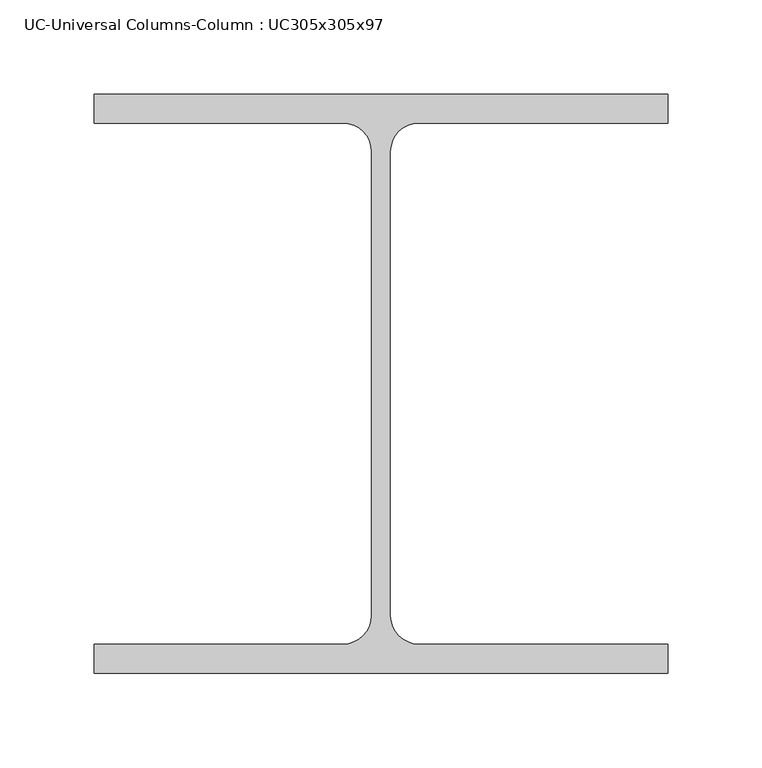
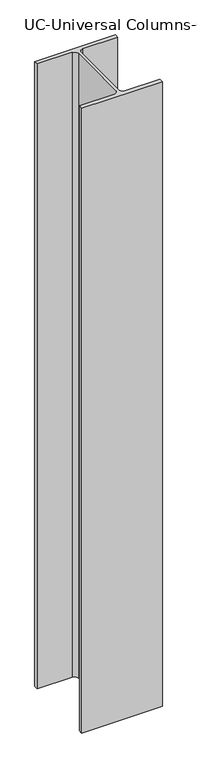
"""IFC4 building model written with IfcOpenShell, lengths in millimetres: column geometry, UC-Universal Columns-Column : UC305x305x97."""

from ifc_helpers import new_model, si_unit, point, frame_2d, origin, origin_with_axes, place, context, project, spatial, polyline, circle_curve, trimmed, segment, composite_curve, outline, extrude, source, transform, mapped, element, save


def uc_universal_columns_column_uc305x305x97_3ae92ab7(model_context):
    return source(origin(), model_context, "Body", "SweptSolid", [
        extrude(outline(composite_curve([segment(polyline([(152.65, 153.95), (152.65, 138.55), (20.15, 138.55)]), True, "CONTINUOUS"), segment(trimmed(circle_curve(frame_2d((20.15, 123.35)), 15.2), [point((20.15, 138.55))], [point((4.95, 123.35))], True, "CARTESIAN"), True, "CONTINUOUS"), segment(polyline([(4.95, 123.35), (4.95, -123.35)]), True, "CONTINUOUS"), segment(trimmed(circle_curve(frame_2d((20.15, -123.35)), 15.2), [point((4.95, -123.35))], [point((20.15, -138.55))], True, "CARTESIAN"), True, "CONTINUOUS"), segment(polyline([(20.15, -138.55), (152.65, -138.55), (152.65, -153.95), (-152.65, -153.95), (-152.65, -138.55), (-20.15, -138.55)]), True, "CONTINUOUS"), segment(trimmed(circle_curve(frame_2d((-20.15, -123.35)), 15.2), [point((-20.15, -138.55))], [point((-4.95, -123.35))], True, "CARTESIAN"), True, "CONTINUOUS"), segment(polyline([(-4.95, -123.35), (-4.95, 123.35)]), True, "CONTINUOUS"), segment(trimmed(circle_curve(frame_2d((-20.15, 123.35)), 15.2), [point((-4.95, 123.35))], [point((-20.15, 138.55))], True, "CARTESIAN"), True, "CONTINUOUS"), segment(polyline([(-20.15, 138.55), (-152.65, 138.55), (-152.65, 153.95), (152.65, 153.95)]), True, "CONTINUOUS")], self_intersect=False)), origin_with_axes(), (0.0, 0.0, 1.0), 2500.0),
    ])


if __name__ == "__main__":
    model = new_model("IFC4")
    model_context = context("Model", 3, world=origin())
    ifc_project = project(units=[si_unit("LENGTHUNIT", "METRE", prefix="MILLI")], contexts=[model_context])
    site = spatial("IfcSite", under=ifc_project)
    building = spatial("IfcBuilding", under=site)
    placement = place(None, origin())
    uc_universal_columns_column_uc305x305x97_shape = uc_universal_columns_column_uc305x305x97_3ae92ab7(model_context)
    element("IfcColumn", 1, ObjectType="UC-Universal Columns-Column : UC305x305x97", at=placement, inside=building, context=model_context, shape_type="MappedRepresentation", body=[
        mapped(uc_universal_columns_column_uc305x305x97_shape, transform((0.0, 0.0, 0.0), x_axis=(1.0, 0.0, 0.0), y_axis=(0.0, 1.0, 0.0), z_axis=(0.0, 0.0, 1.0))),
    ])
    save(model, "model.ifc")

# Revit data of these elements
# Project information
#   Project Issue Date = "Issue Date"
#   Project Status = "Project Status"
#   Client Name = "Owner"
#   Project Address = "Enter address here"
#   Project Name = "Project Name"
#   Project Number = "0001"
# Type "UC-Universal Columns-Column : UC305x305x97"
#   Section Name Key = "UC305x305x97"
#   Width = 30.53 cm
#   Web Thickness = 0.99 cm
#   Web Fillet = 1.52 cm
#   Warping Constant = 1560000.0 cm⁶
#   Torsional Moment of Inertia = 91.20 cm⁴
#   Section Area = 123.0 cm²
#   Plastic Modulus weak axis = 726.0 cm³
#   Plastic Modulus strong axis = 1592.0 cm³
#   Nominal Weight = 96.8996 kgf/m
#   Moment of Inertia weak axis = 7308.00 cm⁴
#   Moment of Inertia strong axis = 22249.00 cm⁴
#   Height = 30.79 cm
#   Flange Thickness = 1.54 cm
#   Elastic Modulus weak axis = 479.0 cm³
#   Elastic Modulus strong axis = 1445.0 cm³
#   Centroid Vertical = 15.395 cm
#   Centroid Horizontal = 15.265 cm
#   Bolt Spacing = 14.0 cm
#   Structural Material [instance default] = Metal - Steel 43-275
#   Type Comments = ""
#   Assembly Code = ""
# Element 1 (IfcColumn, "UC-Universal Columns-Column : UC305x305x97")
#   Materials on its faces: "Metal - Steel 43-275"
# Materials
#   "Metal - Steel 43-275": class "Metal", colour RGB 247 247 247, transparency 0, Cost = 0
